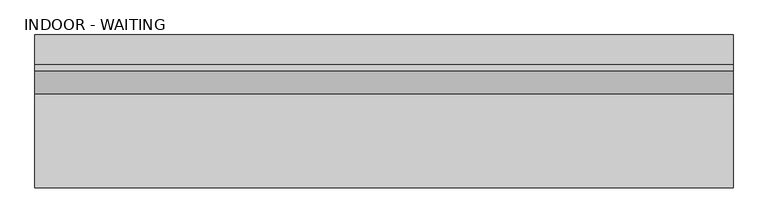
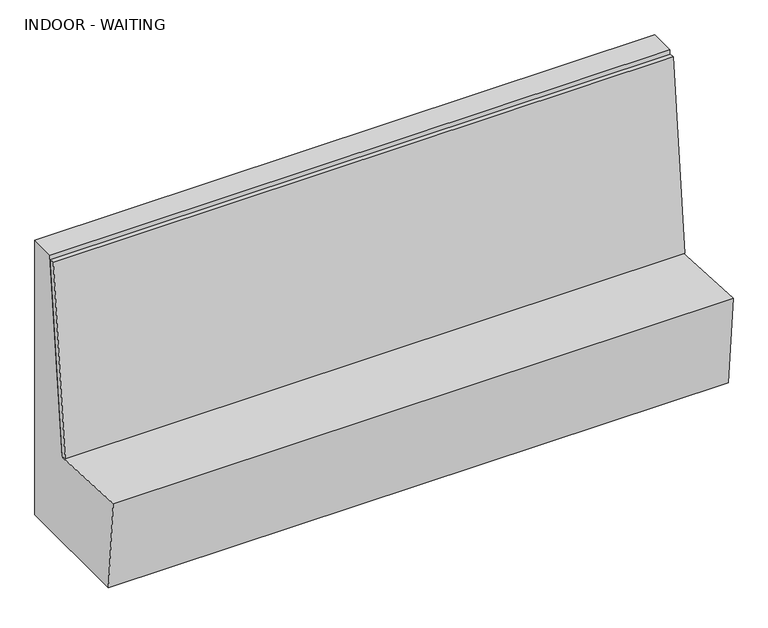
"""IFC4 building model written with IfcOpenShell, lengths in millimetres: furniture geometry, OD_CW_Booth : INDOOR - WAITING."""

import ifcopenshell
import ifcopenshell.guid

model = None  # the IFC model being written
_history = None  # IfcOwnerHistory: only IFC2X3 demands one
_inside = {}  # id of a spatial element -> (the spatial element, [elements in it])
_under = {}  # id of a project, library or spatial element -> (it, [spatial elements below it])
_declared = {}  # id of a project -> (the project, [libraries it declares])
_typed = {}  # id of a type object -> (the type object, [elements of that type])
_made_of = {}  # id of a material, layer set ... -> (it, [elements and type objects made of it])


def new_model(schema):
    """Start an empty IFC model of exactly this schema.

    Asked for "IFC4X3", IfcOpenShell would pick the latest addendum, in which some entities
    have other attributes; the version numbers below select the first issue.
    IFC2X3 requires an IfcOwnerHistory on every rooted entity: one is made here for all.
    """
    global model, _history
    if schema == "IFC4X3":
        model = ifcopenshell.file(schema_version=(4, 3, 0, 0))
    else:
        model = ifcopenshell.file(schema=schema)
    _inside.clear()
    _under.clear()
    _declared.clear()
    _typed.clear()
    _made_of.clear()
    _history = None
    if model.schema == "IFC2X3":
        org = make("IfcOrganization", Name="unknown")
        user = make(
            "IfcPersonAndOrganization",
            ThePerson=make("IfcPerson", FamilyName="unknown"),
            TheOrganization=org,
        )
        app = make(
            "IfcApplication",
            ApplicationDeveloper=org,
            Version="unknown",
            ApplicationFullName="unknown",
            ApplicationIdentifier="unknown",
        )
        _history = make(
            "IfcOwnerHistory",
            OwningUser=user,
            OwningApplication=app,
            ChangeAction="ADDED",
            CreationDate=0,
        )
    return model


def make(cls, **values):
    """One entity of the class cls with the attributes given. An attribute that is None is left unset."""
    return model.create_entity(
        cls, **{name: value for name, value in values.items() if value is not None}
    )


def rooted(cls, **values):
    """An entity with a GlobalId (a new one), such as an element, a storey or a relation."""
    return make(cls, GlobalId=ifcopenshell.guid.new(), OwnerHistory=_history, **values)


def si_unit(unit_type, name, prefix=None):
    """IfcSIUnit, for example si_unit("LENGTHUNIT", "METRE", prefix="MILLI")."""
    return make("IfcSIUnit", UnitType=unit_type, Prefix=prefix, Name=name)


def assignment(units):
    """IfcUnitAssignment: the units of a project."""
    return None if units is None else make("IfcUnitAssignment", Units=units)


def point(xyz):
    """IfcCartesianPoint."""
    return None if xyz is None else make("IfcCartesianPoint", Coordinates=xyz)


def direction(xyz):
    """IfcDirection."""
    return None if xyz is None else make("IfcDirection", DirectionRatios=xyz)


def frame(location, z_axis=None, x_axis=None):
    """IfcAxis2Placement3D, a coordinate frame: its origin and axes. An axis left out is left unset."""
    return make(
        "IfcAxis2Placement3D",
        Location=point(location),
        Axis=direction(z_axis),
        RefDirection=direction(x_axis),
    )


def origin():
    """The frame at (0, 0, 0) with its axes left unset."""
    return frame((0.0, 0.0, 0.0))


def place(relative_to, where):
    """IfcLocalPlacement: puts the frame where relative to a parent placement (None: the world)."""
    return make(
        "IfcLocalPlacement", PlacementRelTo=relative_to, RelativePlacement=where
    )


def context(
    kind, dimensions, precision=None, world=None, true_north=None, identifier=None
):
    """IfcGeometricRepresentationContext, for example the 3D "Model" context."""
    return make(
        "IfcGeometricRepresentationContext",
        ContextIdentifier=identifier,
        ContextType=kind,
        CoordinateSpaceDimension=dimensions,
        Precision=precision,
        WorldCoordinateSystem=world,
        TrueNorth=true_north,
    )


def project(units=None, contexts=None):
    """IfcProject with its units and contexts."""
    return rooted(
        "IfcProject",
        Name="project",
        RepresentationContexts=contexts,
        UnitsInContext=assignment(units),
    )


def spatial(cls, under=None, at=None, **own):
    """A site, building, storey or space (cls), placed at a placement, below another one or the project."""
    s = rooted(cls, ObjectPlacement=at, **own)
    if under is not None:
        _under.setdefault(under.id(), (under, []))[1].append(s)
    return s


def polyline(points):
    """IfcPolyline through the points."""
    return make("IfcPolyline", Points=[point(p) for p in points])


def outline(outer, holes=None, kind="AREA"):
    """IfcArbitraryClosedProfileDef: a profile drawn as a closed curve; with holes, ...WithVoids."""
    if holes is None:
        return make("IfcArbitraryClosedProfileDef", ProfileType=kind, OuterCurve=outer)
    return make(
        "IfcArbitraryProfileDefWithVoids",
        ProfileType=kind,
        OuterCurve=outer,
        InnerCurves=holes,
    )


def extrude(swept, where, along, depth):
    """IfcExtrudedAreaSolid: the profile swept, set in the frame where, extruded along a direction by depth."""
    return make(
        "IfcExtrudedAreaSolid",
        SweptArea=swept,
        Position=where,
        ExtrudedDirection=direction(along),
        Depth=depth,
    )


def shape(context_of_items, identifier, shape_type, items):
    """IfcShapeRepresentation: the items that make up one representation, for example the "Body"."""
    return make(
        "IfcShapeRepresentation",
        ContextOfItems=context_of_items,
        RepresentationIdentifier=identifier,
        RepresentationType=shape_type,
        Items=items,
    )


def source(mapping_origin, context_of_items, identifier, shape_type, items):
    """IfcRepresentationMap: a shape defined once, which mapped items show again and again."""
    return make(
        "IfcRepresentationMap",
        MappingOrigin=mapping_origin,
        MappedRepresentation=shape(context_of_items, identifier, shape_type, items),
    )


def transform(
    local_origin,
    x_axis=None,
    y_axis=None,
    z_axis=None,
    scale=None,
    scale2=None,
    scale3=None,
    uniform=True,
):
    """IfcCartesianTransformationOperator3D, or its non-uniform kind. x_axis, y_axis, z_axis: its Axis1, 2, 3."""
    if uniform:
        return make(
            "IfcCartesianTransformationOperator3D",
            Axis1=direction(x_axis),
            Axis2=direction(y_axis),
            LocalOrigin=point(local_origin),
            Scale=scale,
            Axis3=direction(z_axis),
        )
    return make(
        "IfcCartesianTransformationOperator3DnonUniform",
        Axis1=direction(x_axis),
        Axis2=direction(y_axis),
        LocalOrigin=point(local_origin),
        Scale=scale,
        Axis3=direction(z_axis),
        Scale2=scale2,
        Scale3=scale3,
    )


def mapped(mapping_source, mapping_target):
    """IfcMappedItem: shows the shape of a source again, moved by a transform."""
    return make(
        "IfcMappedItem", MappingSource=mapping_source, MappingTarget=mapping_target
    )


def made_of(thing, what):
    """Note that an element or type object is made of a material, layer set ...; save() writes the relation."""
    if what is not None:
        _made_of.setdefault(what.id(), (what, []))[1].append(thing)
    return thing


def element(
    cls,
    number,
    at=None,
    inside=None,
    cuts=None,
    type_object=None,
    material=None,
    context=None,
    identifier="Body",
    shape_type=None,
    held_by="IfcProductDefinitionShape",
    body=None,
    shapes=None,
    **own,
):
    """One element of the class cls, such as IfcWall. Its Tag is "e" and its number.

    at: its placement. inside: the storey or other place that contains it. cuts: it is an
    opening in that element (IfcRelVoidsElement). A single representation is given by context,
    identifier, shape_type and body (its items); several are given by shapes. held_by: the class
    of the entity that holds the representations. save() writes the other relations.
    """
    e = rooted(cls, Tag="e%d" % number, ObjectPlacement=at, **own)
    if body is not None:
        shapes = [shape(context, identifier, shape_type, body)]
    if shapes is not None:
        e.Representation = make(held_by, Representations=shapes)
    if inside is not None:
        _inside.setdefault(inside.id(), (inside, []))[1].append(e)
    if cuts is not None:
        rooted(
            "IfcRelVoidsElement", RelatingBuildingElement=cuts, RelatedOpeningElement=e
        )
    if type_object is not None:
        _typed.setdefault(type_object.id(), (type_object, []))[1].append(e)
    return made_of(e, material)


def aggregate(whole, parts):
    """IfcRelAggregates: a whole, such as a stair, and the parts it consists of."""
    return rooted("IfcRelAggregates", RelatingObject=whole, RelatedObjects=parts)


def save(model, path):
    """Write the relations noted so far, then the file.

    IfcRelAggregates (storeys below a building ...), IfcRelContainedInSpatialStructure (elements
    in a storey), IfcRelDefinesByType, IfcRelAssociatesMaterial and IfcRelDeclares: one each for
    every whole, place, type object, material and project.
    """
    for whole, parts in _under.values():
        aggregate(whole, parts)
    for where, things in _inside.values():
        rooted(
            "IfcRelContainedInSpatialStructure",
            RelatedElements=things,
            RelatingStructure=where,
        )
    for kind, things in _typed.values():
        rooted("IfcRelDefinesByType", RelatedObjects=things, RelatingType=kind)
    for what, things in _made_of.values():
        rooted("IfcRelAssociatesMaterial", RelatedObjects=things, RelatingMaterial=what)
    for by, libraries in _declared.values():
        rooted("IfcRelDeclares", RelatingContext=by, RelatedDefinitions=libraries)
    model.write(path)


def indoor_waiting_de4477bf(model_context):
    return source(origin(), model_context, "Body", "SweptSolid", [
        extrude(outline(polyline([(0.0, 2981.9570278), (25.4, 2981.9570278), (25.4, 0.0), (0.0, 0.0), (0.0, 2981.9570278)])), frame((3000.6947327, 358.2049359, 438.8309433), z_axis=(0.0, 0.10452846326765197, 0.9945218953682735), x_axis=(0.0, 0.9945218953682735, -0.10452846326765197)), (0.0, 0.0, 1.0), 944.7333479),
        extrude(outline(polyline([(609.6, 1397.0), (609.6, 0.0), (-3.4100193, 0.0), (-43.0849153, 453.4861359), (382.9385128, 431.1591941), (484.4524721, 1397.0), (609.6, 1397.0)])), frame((18.7377049, 0.0, 0.0), z_axis=(1.0, 0.0, 0.0), x_axis=(0.0, 1.0, 0.0)), (0.0, 0.0, 1.0), 2981.9570278),
    ])


if __name__ == "__main__":
    model = new_model("IFC4")
    model_context = context("Model", 3, world=origin())
    ifc_project = project(units=[si_unit("LENGTHUNIT", "METRE", prefix="MILLI")], contexts=[model_context])
    site = spatial("IfcSite", under=ifc_project)
    building = spatial("IfcBuilding", under=site)
    placement = place(None, origin())
    indoor_waiting_shape = indoor_waiting_de4477bf(model_context)
    element("IfcFurniture", 1, ObjectType="OD_CW_Booth : INDOOR - WAITING", at=placement, inside=building, context=model_context, shape_type="MappedRepresentation", body=[
        mapped(indoor_waiting_shape, transform((0.0, 0.0, 0.0), x_axis=(1.0, 0.0, 0.0), y_axis=(0.0, 1.0, 0.0), z_axis=(0.0, 0.0, 1.0))),
    ])
    save(model, "model.ifc")

# Revit data of these elements
# Type "OD_CW_Booth : INDOOR - WAITING"
#   Width = 4' - 0"
#   OD_CW_Width [instance default] = 2' - 10"
#   OD_CW_Length [instance default] = 26' - 1 83/256"
#   OD_CW_Height [instance default] = 2' - 3"
#   Height = 3' - 0"
#   Depth = 2' - 0"
#   Seating Count [instance default] = 10
#   back = Casework-oakfire
#   OD_CW_Material_Front Panel [instance default] = none
#   OD_CW_Material_Body [instance default] = none
# Element 1 (IfcFurniture, "OD_CW_Booth : INDOOR - WAITING")
#   OD_CW_Length = 9' - 9.39988"
#   Seating Count = 4
#   OD_CW_Material_Body = WOOD-OAKFIRE
#   Materials on its faces: "WOOD-OAKFIRE", "Casework-oakfire"
# Materials
#   "Casework-oakfire": class "Miscellaneous", colour RGB 164 164 164, transparency 0, Cost = 0
#   "WOOD-OAKFIRE": class "Wood", colour RGB 198 202 183, transparency 0, Description = "Generic wood", Cost = 0
